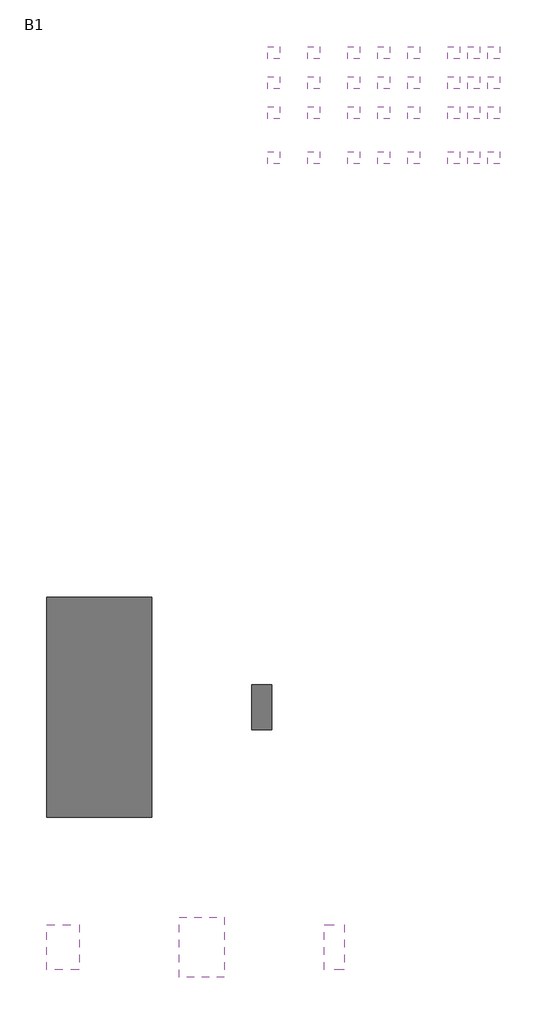
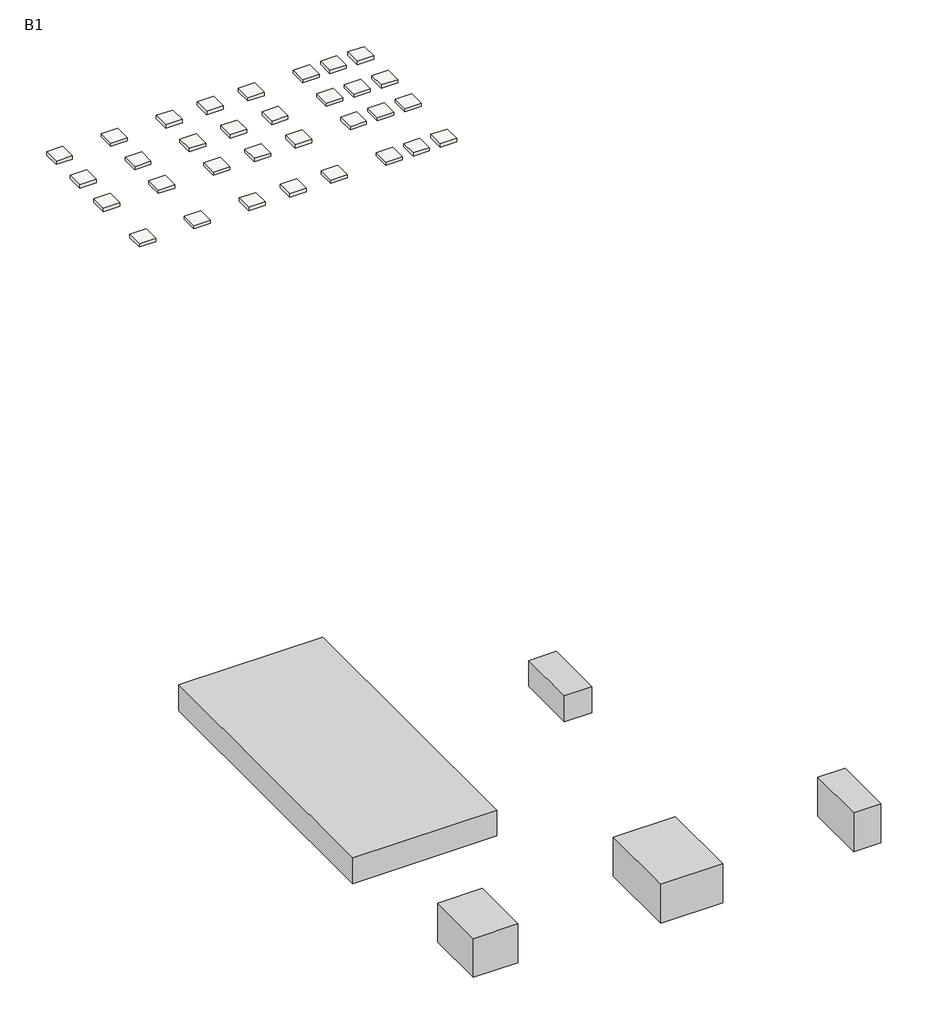
# One storey: 32 slabs, 5 proxies.
"""IFC4 building model written with IfcOpenShell, lengths in millimetres."""

import ifcopenshell
import ifcopenshell.guid

model = None  # the IFC model being written
_history = None  # IfcOwnerHistory: only IFC2X3 demands one
_inside = {}  # id of a spatial element -> (the spatial element, [elements in it])
_under = {}  # id of a project, library or spatial element -> (it, [spatial elements below it])
_declared = {}  # id of a project -> (the project, [libraries it declares])
_typed = {}  # id of a type object -> (the type object, [elements of that type])
_made_of = {}  # id of a material, layer set ... -> (it, [elements and type objects made of it])


def new_model(schema):
    """Start an empty IFC model of exactly this schema.

    Asked for "IFC4X3", IfcOpenShell would pick the latest addendum, in which some entities
    have other attributes; the version numbers below select the first issue.
    IFC2X3 requires an IfcOwnerHistory on every rooted entity: one is made here for all.
    """
    global model, _history
    if schema == "IFC4X3":
        model = ifcopenshell.file(schema_version=(4, 3, 0, 0))
    else:
        model = ifcopenshell.file(schema=schema)
    _inside.clear()
    _under.clear()
    _declared.clear()
    _typed.clear()
    _made_of.clear()
    _history = None
    if model.schema == "IFC2X3":
        org = make("IfcOrganization", Name="unknown")
        user = make(
            "IfcPersonAndOrganization",
            ThePerson=make("IfcPerson", FamilyName="unknown"),
            TheOrganization=org,
        )
        app = make(
            "IfcApplication",
            ApplicationDeveloper=org,
            Version="unknown",
            ApplicationFullName="unknown",
            ApplicationIdentifier="unknown",
        )
        _history = make(
            "IfcOwnerHistory",
            OwningUser=user,
            OwningApplication=app,
            ChangeAction="ADDED",
            CreationDate=0,
        )
    return model


def make(cls, **values):
    """One entity of the class cls with the attributes given. An attribute that is None is left unset."""
    return model.create_entity(
        cls, **{name: value for name, value in values.items() if value is not None}
    )


def rooted(cls, **values):
    """An entity with a GlobalId (a new one), such as an element, a storey or a relation."""
    return make(cls, GlobalId=ifcopenshell.guid.new(), OwnerHistory=_history, **values)


def si_unit(unit_type, name, prefix=None):
    """IfcSIUnit, for example si_unit("LENGTHUNIT", "METRE", prefix="MILLI")."""
    return make("IfcSIUnit", UnitType=unit_type, Prefix=prefix, Name=name)


def assignment(units):
    """IfcUnitAssignment: the units of a project."""
    return None if units is None else make("IfcUnitAssignment", Units=units)


def point(xyz):
    """IfcCartesianPoint."""
    return None if xyz is None else make("IfcCartesianPoint", Coordinates=xyz)


def direction(xyz):
    """IfcDirection."""
    return None if xyz is None else make("IfcDirection", DirectionRatios=xyz)


def frame(location, z_axis=None, x_axis=None):
    """IfcAxis2Placement3D, a coordinate frame: its origin and axes. An axis left out is left unset."""
    return make(
        "IfcAxis2Placement3D",
        Location=point(location),
        Axis=direction(z_axis),
        RefDirection=direction(x_axis),
    )


def origin():
    """The frame at (0, 0, 0) with its axes left unset."""
    return frame((0.0, 0.0, 0.0))


def origin_with_axes():
    """The frame at (0, 0, 0) with the z axis (0, 0, 1) and the x axis (1, 0, 0) written out."""
    return frame((0.0, 0.0, 0.0), z_axis=(0.0, 0.0, 1.0), x_axis=(1.0, 0.0, 0.0))


def place(relative_to, where):
    """IfcLocalPlacement: puts the frame where relative to a parent placement (None: the world)."""
    return make(
        "IfcLocalPlacement", PlacementRelTo=relative_to, RelativePlacement=where
    )


def context(
    kind, dimensions, precision=None, world=None, true_north=None, identifier=None
):
    """IfcGeometricRepresentationContext, for example the 3D "Model" context."""
    return make(
        "IfcGeometricRepresentationContext",
        ContextIdentifier=identifier,
        ContextType=kind,
        CoordinateSpaceDimension=dimensions,
        Precision=precision,
        WorldCoordinateSystem=world,
        TrueNorth=true_north,
    )


def project(units=None, contexts=None):
    """IfcProject with its units and contexts."""
    return rooted(
        "IfcProject",
        Name="project",
        RepresentationContexts=contexts,
        UnitsInContext=assignment(units),
    )


def spatial(cls, under=None, at=None, **own):
    """A site, building, storey or space (cls), placed at a placement, below another one or the project."""
    s = rooted(cls, ObjectPlacement=at, **own)
    if under is not None:
        _under.setdefault(under.id(), (under, []))[1].append(s)
    return s


def polyline(points):
    """IfcPolyline through the points."""
    return make("IfcPolyline", Points=[point(p) for p in points])


def outline(outer, holes=None, kind="AREA"):
    """IfcArbitraryClosedProfileDef: a profile drawn as a closed curve; with holes, ...WithVoids."""
    if holes is None:
        return make("IfcArbitraryClosedProfileDef", ProfileType=kind, OuterCurve=outer)
    return make(
        "IfcArbitraryProfileDefWithVoids",
        ProfileType=kind,
        OuterCurve=outer,
        InnerCurves=holes,
    )


def extrude(swept, where, along, depth):
    """IfcExtrudedAreaSolid: the profile swept, set in the frame where, extruded along a direction by depth."""
    return make(
        "IfcExtrudedAreaSolid",
        SweptArea=swept,
        Position=where,
        ExtrudedDirection=direction(along),
        Depth=depth,
    )


def shape(context_of_items, identifier, shape_type, items):
    """IfcShapeRepresentation: the items that make up one representation, for example the "Body"."""
    return make(
        "IfcShapeRepresentation",
        ContextOfItems=context_of_items,
        RepresentationIdentifier=identifier,
        RepresentationType=shape_type,
        Items=items,
    )


def source(mapping_origin, context_of_items, identifier, shape_type, items):
    """IfcRepresentationMap: a shape defined once, which mapped items show again and again."""
    return make(
        "IfcRepresentationMap",
        MappingOrigin=mapping_origin,
        MappedRepresentation=shape(context_of_items, identifier, shape_type, items),
    )


def transform(
    local_origin,
    x_axis=None,
    y_axis=None,
    z_axis=None,
    scale=None,
    scale2=None,
    scale3=None,
    uniform=True,
):
    """IfcCartesianTransformationOperator3D, or its non-uniform kind. x_axis, y_axis, z_axis: its Axis1, 2, 3."""
    if uniform:
        return make(
            "IfcCartesianTransformationOperator3D",
            Axis1=direction(x_axis),
            Axis2=direction(y_axis),
            LocalOrigin=point(local_origin),
            Scale=scale,
            Axis3=direction(z_axis),
        )
    return make(
        "IfcCartesianTransformationOperator3DnonUniform",
        Axis1=direction(x_axis),
        Axis2=direction(y_axis),
        LocalOrigin=point(local_origin),
        Scale=scale,
        Axis3=direction(z_axis),
        Scale2=scale2,
        Scale3=scale3,
    )


def mapped(mapping_source, mapping_target):
    """IfcMappedItem: shows the shape of a source again, moved by a transform."""
    return make(
        "IfcMappedItem", MappingSource=mapping_source, MappingTarget=mapping_target
    )


def made_of(thing, what):
    """Note that an element or type object is made of a material, layer set ...; save() writes the relation."""
    if what is not None:
        _made_of.setdefault(what.id(), (what, []))[1].append(thing)
    return thing


def element(
    cls,
    number,
    at=None,
    inside=None,
    cuts=None,
    type_object=None,
    material=None,
    context=None,
    identifier="Body",
    shape_type=None,
    held_by="IfcProductDefinitionShape",
    body=None,
    shapes=None,
    **own,
):
    """One element of the class cls, such as IfcWall. Its Tag is "e" and its number.

    at: its placement. inside: the storey or other place that contains it. cuts: it is an
    opening in that element (IfcRelVoidsElement). A single representation is given by context,
    identifier, shape_type and body (its items); several are given by shapes. held_by: the class
    of the entity that holds the representations. save() writes the other relations.
    """
    e = rooted(cls, Tag="e%d" % number, ObjectPlacement=at, **own)
    if body is not None:
        shapes = [shape(context, identifier, shape_type, body)]
    if shapes is not None:
        e.Representation = make(held_by, Representations=shapes)
    if inside is not None:
        _inside.setdefault(inside.id(), (inside, []))[1].append(e)
    if cuts is not None:
        rooted(
            "IfcRelVoidsElement", RelatingBuildingElement=cuts, RelatedOpeningElement=e
        )
    if type_object is not None:
        _typed.setdefault(type_object.id(), (type_object, []))[1].append(e)
    return made_of(e, material)


def aggregate(whole, parts):
    """IfcRelAggregates: a whole, such as a stair, and the parts it consists of."""
    return rooted("IfcRelAggregates", RelatingObject=whole, RelatedObjects=parts)


def save(model, path):
    """Write the relations noted so far, then the file.

    IfcRelAggregates (storeys below a building ...), IfcRelContainedInSpatialStructure (elements
    in a storey), IfcRelDefinesByType, IfcRelAssociatesMaterial and IfcRelDeclares: one each for
    every whole, place, type object, material and project.
    """
    for whole, parts in _under.values():
        aggregate(whole, parts)
    for where, things in _inside.values():
        rooted(
            "IfcRelContainedInSpatialStructure",
            RelatedElements=things,
            RelatingStructure=where,
        )
    for kind, things in _typed.values():
        rooted("IfcRelDefinesByType", RelatedObjects=things, RelatingType=kind)
    for what, things in _made_of.values():
        rooted("IfcRelAssociatesMaterial", RelatedObjects=things, RelatingMaterial=what)
    for by, libraries in _declared.values():
        rooted("IfcRelDeclares", RelatingContext=by, RelatedDefinitions=libraries)
    model.write(path)


def generic_models_1d705098(model_context):
    return source(origin(), model_context, "Body", "SweptSolid", [
        extrude(outline(polyline([(3250.0, 4500.0), (3250.0, -4500.0), (-3250.0, -4500.0), (-3250.0, 4500.0), (3250.0, 4500.0)])), origin_with_axes(), (0.0, 0.0, 1.0), 6000.0),
    ])


def generic_models_399a6151(model_context):
    return source(origin(), model_context, "Body", "SweptSolid", [
        extrude(outline(polyline([(4500.0, 6000.0), (4500.0, -6000.0), (-4500.0, -6000.0), (-4500.0, 6000.0), (4500.0, 6000.0)])), origin_with_axes(), (0.0, 0.0, 1.0), 6000.0),
    ])


def generic_models_29bcd6f9(model_context):
    return source(origin(), model_context, "Body", "SweptSolid", [
        extrude(outline(polyline([(2000.0, 4500.0), (2000.0, -4500.0), (-2000.0, -4500.0), (-2000.0, 4500.0), (2000.0, 4500.0)])), origin_with_axes(), (0.0, 0.0, 1.0), 6000.0),
    ])


def generic_models_a454a2aa(model_context):
    return source(origin(), model_context, "Body", "SweptSolid", [
        extrude(outline(polyline([(10500.0, 22000.0), (10500.0, -22000.0), (-10500.0, -22000.0), (-10500.0, 22000.0), (10500.0, 22000.0)])), origin_with_axes(), (0.0, 0.0, 1.0), 4000.0),
    ])


def generic_models_73802227(model_context):
    return source(origin(), model_context, "Body", "SweptSolid", [
        extrude(outline(polyline([(2000.0, 4500.0), (2000.0, -4500.0), (-2000.0, -4500.0), (-2000.0, 4500.0), (2000.0, 4500.0)])), origin_with_axes(), (0.0, 0.0, 1.0), 4000.0),
    ])


def ft112_footing_rectangular_ft112_2400x2400x500_5fe39465(model_context):
    return source(origin(), model_context, "Body", "SweptSolid", [
        extrude(outline(polyline([(1200.0, 1200.0), (1200.0, -1200.0), (-1200.0, -1200.0), (-1200.0, 1200.0), (1200.0, 1200.0)])), frame((0.0, 0.0, -500.0), z_axis=(0.0, 0.0, 1.0), x_axis=(1.0, 0.0, 0.0)), (0.0, 0.0, 1.0), 500.0),
    ])


model = new_model("IFC4")

# Units and contexts
model_context = context("Model", 3, world=origin())
ifc_project = project(units=[si_unit("LENGTHUNIT", "METRE", prefix="MILLI")], contexts=[model_context])

# Site, building, storey
site = spatial("IfcSite", under=ifc_project)
building = spatial("IfcBuilding", under=site)
storey = spatial("IfcBuildingStorey", under=building, Name="B1", Elevation=-4000.0)

# Proxies
placement = place(None, origin())
generic_models_shape = generic_models_1d705098(model_context)
element("IfcBuildingElementProxy", 1, Name="Space Planning Box_hec : Space Planning Box_hec", ObjectType="Space Planning Box_hec : Space Planning Box_hec", at=placement, inside=storey, context=model_context, shape_type="MappedRepresentation", body=[
    mapped(generic_models_shape, transform((3250.0, 6000.0, 0.0), x_axis=(1.0, 0.0, 0.0), y_axis=(0.0, 1.0, 0.0), z_axis=(0.0, 0.0, 1.0))),
])
generic_models_2_shape = generic_models_399a6151(model_context)
element("IfcBuildingElementProxy", 2, Name="Space Planning Box_hec : Space Planning Box_hec", ObjectType="Space Planning Box_hec : Space Planning Box_hec", at=placement, inside=storey, context=model_context, shape_type="MappedRepresentation", body=[
    mapped(generic_models_2_shape, transform((31000.0, 6000.0, 0.0), x_axis=(1.0, 0.0, 0.0), y_axis=(0.0, 1.0, 0.0), z_axis=(0.0, 0.0, 1.0))),
])
generic_models_3_shape = generic_models_29bcd6f9(model_context)
element("IfcBuildingElementProxy", 3, Name="Space Planning Box_hec : Space Planning Box_hec", ObjectType="Space Planning Box_hec : Space Planning Box_hec", at=placement, inside=storey, context=model_context, shape_type="MappedRepresentation", body=[
    mapped(generic_models_3_shape, transform((57500.0, 6000.0, 0.0), x_axis=(1.0, 0.0, 0.0), y_axis=(0.0, 1.0, 0.0), z_axis=(0.0, 0.0, 1.0))),
])
generic_models_4_shape = generic_models_a454a2aa(model_context)
element("IfcBuildingElementProxy", 4, Name="Space Planning Box_hec : Space Planning Box_hec", ObjectType="Space Planning Box_hec : Space Planning Box_hec", at=placement, inside=storey, context=model_context, shape_type="MappedRepresentation", body=[
    mapped(generic_models_4_shape, transform((10500.0, 54000.0, -4000.0), x_axis=(1.0, 0.0, 0.0), y_axis=(0.0, 1.0, 0.0), z_axis=(0.0, 0.0, 1.0))),
])
generic_models_5_shape = generic_models_73802227(model_context)
element("IfcBuildingElementProxy", 5, Name="Space Planning Box_hec : Space Planning Box_hec", ObjectType="Space Planning Box_hec : Space Planning Box_hec", at=placement, inside=storey, context=model_context, shape_type="MappedRepresentation", body=[
    mapped(generic_models_5_shape, transform((43000.0, 54000.0, -4000.0), x_axis=(1.0, 0.0, 0.0), y_axis=(0.0, 1.0, 0.0), z_axis=(0.0, 0.0, 1.0))),
])

# Slabs
ft112_footing_rectangular_ft112_2400x2400x500_shape = ft112_footing_rectangular_ft112_2400x2400x500_5fe39465(model_context)
element("IfcSlab", 6, ObjectType="FT112-Footing-Rectangular : FT112_2400x2400x500", at=placement, inside=storey, context=model_context, shape_type="MappedRepresentation", body=[
    mapped(ft112_footing_rectangular_ft112_2400x2400x500_shape, transform((45459.6521483, 184923.8614395, 0.0), x_axis=(1.0, 0.0, 0.0), y_axis=(0.0, 1.0, 0.0), z_axis=(0.0, 0.0, 1.0))),
])
element("IfcSlab", 7, ObjectType="FT112-Footing-Rectangular : FT112_2400x2400x500", at=placement, inside=storey, context=model_context, shape_type="MappedRepresentation", body=[
    mapped(ft112_footing_rectangular_ft112_2400x2400x500_shape, transform((45459.6521483, 178923.8614395, 0.0), x_axis=(1.0, 0.0, 0.0), y_axis=(0.0, 1.0, 0.0), z_axis=(0.0, 0.0, 1.0))),
])
element("IfcSlab", 8, ObjectType="FT112-Footing-Rectangular : FT112_2400x2400x500", at=placement, inside=storey, context=model_context, shape_type="MappedRepresentation", body=[
    mapped(ft112_footing_rectangular_ft112_2400x2400x500_shape, transform((45459.6521483, 172923.8614395, 0.0), x_axis=(1.0, 0.0, 0.0), y_axis=(0.0, 1.0, 0.0), z_axis=(0.0, 0.0, 1.0))),
])
element("IfcSlab", 9, ObjectType="FT112-Footing-Rectangular : FT112_2400x2400x500", at=placement, inside=storey, context=model_context, shape_type="MappedRepresentation", body=[
    mapped(ft112_footing_rectangular_ft112_2400x2400x500_shape, transform((45459.6521483, 163923.8614395, 0.0), x_axis=(1.0, 0.0, 0.0), y_axis=(0.0, 1.0, 0.0), z_axis=(0.0, 0.0, 1.0))),
])
element("IfcSlab", 10, ObjectType="FT112-Footing-Rectangular : FT112_2400x2400x500", at=placement, inside=storey, context=model_context, shape_type="MappedRepresentation", body=[
    mapped(ft112_footing_rectangular_ft112_2400x2400x500_shape, transform((53459.6521483, 184923.8614395, 0.0), x_axis=(1.0, 0.0, 0.0), y_axis=(0.0, 1.0, 0.0), z_axis=(0.0, 0.0, 1.0))),
])
element("IfcSlab", 11, ObjectType="FT112-Footing-Rectangular : FT112_2400x2400x500", at=placement, inside=storey, context=model_context, shape_type="MappedRepresentation", body=[
    mapped(ft112_footing_rectangular_ft112_2400x2400x500_shape, transform((53459.6521483, 178923.8614395, 0.0), x_axis=(1.0, 0.0, 0.0), y_axis=(0.0, 1.0, 0.0), z_axis=(0.0, 0.0, 1.0))),
])
element("IfcSlab", 12, ObjectType="FT112-Footing-Rectangular : FT112_2400x2400x500", at=placement, inside=storey, context=model_context, shape_type="MappedRepresentation", body=[
    mapped(ft112_footing_rectangular_ft112_2400x2400x500_shape, transform((53459.6521483, 172923.8614395, 0.0), x_axis=(1.0, 0.0, 0.0), y_axis=(0.0, 1.0, 0.0), z_axis=(0.0, 0.0, 1.0))),
])
element("IfcSlab", 13, ObjectType="FT112-Footing-Rectangular : FT112_2400x2400x500", at=placement, inside=storey, context=model_context, shape_type="MappedRepresentation", body=[
    mapped(ft112_footing_rectangular_ft112_2400x2400x500_shape, transform((53459.6521483, 163923.8614395, 0.0), x_axis=(1.0, 0.0, 0.0), y_axis=(0.0, 1.0, 0.0), z_axis=(0.0, 0.0, 1.0))),
])
element("IfcSlab", 14, ObjectType="FT112-Footing-Rectangular : FT112_2400x2400x500", at=placement, inside=storey, context=model_context, shape_type="MappedRepresentation", body=[
    mapped(ft112_footing_rectangular_ft112_2400x2400x500_shape, transform((61459.6521483, 184923.8614395, 0.0), x_axis=(1.0, 0.0, 0.0), y_axis=(0.0, 1.0, 0.0), z_axis=(0.0, 0.0, 1.0))),
])
element("IfcSlab", 15, ObjectType="FT112-Footing-Rectangular : FT112_2400x2400x500", at=placement, inside=storey, context=model_context, shape_type="MappedRepresentation", body=[
    mapped(ft112_footing_rectangular_ft112_2400x2400x500_shape, transform((61459.6521483, 178923.8614395, 0.0), x_axis=(1.0, 0.0, 0.0), y_axis=(0.0, 1.0, 0.0), z_axis=(0.0, 0.0, 1.0))),
])
element("IfcSlab", 16, ObjectType="FT112-Footing-Rectangular : FT112_2400x2400x500", at=placement, inside=storey, context=model_context, shape_type="MappedRepresentation", body=[
    mapped(ft112_footing_rectangular_ft112_2400x2400x500_shape, transform((61459.6521483, 172923.8614395, 0.0), x_axis=(1.0, 0.0, 0.0), y_axis=(0.0, 1.0, 0.0), z_axis=(0.0, 0.0, 1.0))),
])
element("IfcSlab", 17, ObjectType="FT112-Footing-Rectangular : FT112_2400x2400x500", at=placement, inside=storey, context=model_context, shape_type="MappedRepresentation", body=[
    mapped(ft112_footing_rectangular_ft112_2400x2400x500_shape, transform((61459.6521483, 163923.8614395, 0.0), x_axis=(1.0, 0.0, 0.0), y_axis=(0.0, 1.0, 0.0), z_axis=(0.0, 0.0, 1.0))),
])
element("IfcSlab", 18, ObjectType="FT112-Footing-Rectangular : FT112_2400x2400x500", at=placement, inside=storey, context=model_context, shape_type="MappedRepresentation", body=[
    mapped(ft112_footing_rectangular_ft112_2400x2400x500_shape, transform((67459.6521483, 184923.8614395, 0.0), x_axis=(1.0, 0.0, 0.0), y_axis=(0.0, 1.0, 0.0), z_axis=(0.0, 0.0, 1.0))),
])
element("IfcSlab", 19, ObjectType="FT112-Footing-Rectangular : FT112_2400x2400x500", at=placement, inside=storey, context=model_context, shape_type="MappedRepresentation", body=[
    mapped(ft112_footing_rectangular_ft112_2400x2400x500_shape, transform((67459.6521483, 178923.8614395, 0.0), x_axis=(1.0, 0.0, 0.0), y_axis=(0.0, 1.0, 0.0), z_axis=(0.0, 0.0, 1.0))),
])
element("IfcSlab", 20, ObjectType="FT112-Footing-Rectangular : FT112_2400x2400x500", at=placement, inside=storey, context=model_context, shape_type="MappedRepresentation", body=[
    mapped(ft112_footing_rectangular_ft112_2400x2400x500_shape, transform((67459.6521483, 172923.8614395, 0.0), x_axis=(1.0, 0.0, 0.0), y_axis=(0.0, 1.0, 0.0), z_axis=(0.0, 0.0, 1.0))),
])
element("IfcSlab", 21, ObjectType="FT112-Footing-Rectangular : FT112_2400x2400x500", at=placement, inside=storey, context=model_context, shape_type="MappedRepresentation", body=[
    mapped(ft112_footing_rectangular_ft112_2400x2400x500_shape, transform((67459.6521483, 163923.8614395, 0.0), x_axis=(1.0, 0.0, 0.0), y_axis=(0.0, 1.0, 0.0), z_axis=(0.0, 0.0, 1.0))),
])
element("IfcSlab", 22, ObjectType="FT112-Footing-Rectangular : FT112_2400x2400x500", at=placement, inside=storey, context=model_context, shape_type="MappedRepresentation", body=[
    mapped(ft112_footing_rectangular_ft112_2400x2400x500_shape, transform((73459.6521483, 184923.8614395, 0.0), x_axis=(1.0, 0.0, 0.0), y_axis=(0.0, 1.0, 0.0), z_axis=(0.0, 0.0, 1.0))),
])
element("IfcSlab", 23, ObjectType="FT112-Footing-Rectangular : FT112_2400x2400x500", at=placement, inside=storey, context=model_context, shape_type="MappedRepresentation", body=[
    mapped(ft112_footing_rectangular_ft112_2400x2400x500_shape, transform((73459.6521483, 178923.8614395, 0.0), x_axis=(1.0, 0.0, 0.0), y_axis=(0.0, 1.0, 0.0), z_axis=(0.0, 0.0, 1.0))),
])
element("IfcSlab", 24, ObjectType="FT112-Footing-Rectangular : FT112_2400x2400x500", at=placement, inside=storey, context=model_context, shape_type="MappedRepresentation", body=[
    mapped(ft112_footing_rectangular_ft112_2400x2400x500_shape, transform((73459.6521483, 172923.8614395, 0.0), x_axis=(1.0, 0.0, 0.0), y_axis=(0.0, 1.0, 0.0), z_axis=(0.0, 0.0, 1.0))),
])
element("IfcSlab", 25, ObjectType="FT112-Footing-Rectangular : FT112_2400x2400x500", at=placement, inside=storey, context=model_context, shape_type="MappedRepresentation", body=[
    mapped(ft112_footing_rectangular_ft112_2400x2400x500_shape, transform((73459.6521483, 163923.8614395, 0.0), x_axis=(1.0, 0.0, 0.0), y_axis=(0.0, 1.0, 0.0), z_axis=(0.0, 0.0, 1.0))),
])
element("IfcSlab", 26, ObjectType="FT112-Footing-Rectangular : FT112_2400x2400x500", at=placement, inside=storey, context=model_context, shape_type="MappedRepresentation", body=[
    mapped(ft112_footing_rectangular_ft112_2400x2400x500_shape, transform((81459.6521483, 184923.8614395, 0.0), x_axis=(1.0, 0.0, 0.0), y_axis=(0.0, 1.0, 0.0), z_axis=(0.0, 0.0, 1.0))),
])
element("IfcSlab", 27, ObjectType="FT112-Footing-Rectangular : FT112_2400x2400x500", at=placement, inside=storey, context=model_context, shape_type="MappedRepresentation", body=[
    mapped(ft112_footing_rectangular_ft112_2400x2400x500_shape, transform((81459.6521483, 178923.8614395, 0.0), x_axis=(1.0, 0.0, 0.0), y_axis=(0.0, 1.0, 0.0), z_axis=(0.0, 0.0, 1.0))),
])
element("IfcSlab", 28, ObjectType="FT112-Footing-Rectangular : FT112_2400x2400x500", at=placement, inside=storey, context=model_context, shape_type="MappedRepresentation", body=[
    mapped(ft112_footing_rectangular_ft112_2400x2400x500_shape, transform((81459.6521483, 172923.8614395, 0.0), x_axis=(1.0, 0.0, 0.0), y_axis=(0.0, 1.0, 0.0), z_axis=(0.0, 0.0, 1.0))),
])
element("IfcSlab", 29, ObjectType="FT112-Footing-Rectangular : FT112_2400x2400x500", at=placement, inside=storey, context=model_context, shape_type="MappedRepresentation", body=[
    mapped(ft112_footing_rectangular_ft112_2400x2400x500_shape, transform((81459.6521483, 163923.8614395, 0.0), x_axis=(1.0, 0.0, 0.0), y_axis=(0.0, 1.0, 0.0), z_axis=(0.0, 0.0, 1.0))),
])
element("IfcSlab", 30, ObjectType="FT112-Footing-Rectangular : FT112_2400x2400x500", at=placement, inside=storey, context=model_context, shape_type="MappedRepresentation", body=[
    mapped(ft112_footing_rectangular_ft112_2400x2400x500_shape, transform((85459.6521483, 184923.8614395, 0.0), x_axis=(1.0, 0.0, 0.0), y_axis=(0.0, 1.0, 0.0), z_axis=(0.0, 0.0, 1.0))),
])
element("IfcSlab", 31, ObjectType="FT112-Footing-Rectangular : FT112_2400x2400x500", at=placement, inside=storey, context=model_context, shape_type="MappedRepresentation", body=[
    mapped(ft112_footing_rectangular_ft112_2400x2400x500_shape, transform((85459.6521483, 178923.8614395, 0.0), x_axis=(1.0, 0.0, 0.0), y_axis=(0.0, 1.0, 0.0), z_axis=(0.0, 0.0, 1.0))),
])
element("IfcSlab", 32, ObjectType="FT112-Footing-Rectangular : FT112_2400x2400x500", at=placement, inside=storey, context=model_context, shape_type="MappedRepresentation", body=[
    mapped(ft112_footing_rectangular_ft112_2400x2400x500_shape, transform((85459.6521483, 172923.8614395, 0.0), x_axis=(1.0, 0.0, 0.0), y_axis=(0.0, 1.0, 0.0), z_axis=(0.0, 0.0, 1.0))),
])
element("IfcSlab", 33, ObjectType="FT112-Footing-Rectangular : FT112_2400x2400x500", at=placement, inside=storey, context=model_context, shape_type="MappedRepresentation", body=[
    mapped(ft112_footing_rectangular_ft112_2400x2400x500_shape, transform((85459.6521483, 163923.8614395, 0.0), x_axis=(1.0, 0.0, 0.0), y_axis=(0.0, 1.0, 0.0), z_axis=(0.0, 0.0, 1.0))),
])
element("IfcSlab", 34, ObjectType="FT112-Footing-Rectangular : FT112_2400x2400x500", at=placement, inside=storey, context=model_context, shape_type="MappedRepresentation", body=[
    mapped(ft112_footing_rectangular_ft112_2400x2400x500_shape, transform((89459.6521483, 184923.8614395, 0.0), x_axis=(1.0, 0.0, 0.0), y_axis=(0.0, 1.0, 0.0), z_axis=(0.0, 0.0, 1.0))),
])
element("IfcSlab", 35, ObjectType="FT112-Footing-Rectangular : FT112_2400x2400x500", at=placement, inside=storey, context=model_context, shape_type="MappedRepresentation", body=[
    mapped(ft112_footing_rectangular_ft112_2400x2400x500_shape, transform((89459.6521483, 178923.8614395, 0.0), x_axis=(1.0, 0.0, 0.0), y_axis=(0.0, 1.0, 0.0), z_axis=(0.0, 0.0, 1.0))),
])
element("IfcSlab", 36, ObjectType="FT112-Footing-Rectangular : FT112_2400x2400x500", at=placement, inside=storey, context=model_context, shape_type="MappedRepresentation", body=[
    mapped(ft112_footing_rectangular_ft112_2400x2400x500_shape, transform((89459.6521483, 172923.8614395, 0.0), x_axis=(1.0, 0.0, 0.0), y_axis=(0.0, 1.0, 0.0), z_axis=(0.0, 0.0, 1.0))),
])
element("IfcSlab", 37, ObjectType="FT112-Footing-Rectangular : FT112_2400x2400x500", at=placement, inside=storey, context=model_context, shape_type="MappedRepresentation", body=[
    mapped(ft112_footing_rectangular_ft112_2400x2400x500_shape, transform((89459.6521483, 163923.8614395, 0.0), x_axis=(1.0, 0.0, 0.0), y_axis=(0.0, 1.0, 0.0), z_axis=(0.0, 0.0, 1.0))),
])

save(model, "model.ifc")

# Revit data of these elements
# Project information
#   Building Name = "MAIN GATE SECURITY BUILDING"
#   Project Status = "Project Status"
#   Client Name = "현대엔지니어링"
#   Project Address = "서울시 종로구 율곡로 75(계동)"
#   Project Name = "Therma Visayas Energy Project"
#   Project Number = "-"
# Grids (mm)
#   "A": line (45459.652, 190234.526) -> (45459.652, 152139.384)
#   "B": line (53459.652, 190234.526) -> (53459.652, 152139.384)
#   "C": line (61459.652, 190234.526) -> (61459.652, 152139.384)
#   "D": line (67459.652, 190234.526) -> (67459.652, 152139.384)
#   "E": line (73459.652, 190234.526) -> (73459.652, 152139.384)
#   "F": line (81459.652, 190234.526) -> (81459.652, 152139.384)
#   "G": line (85459.652, 190234.526) -> (85459.652, 152139.384)
#   "H": line (89459.652, 190234.526) -> (89459.652, 152139.384)
#   "4": line (39389.066, 184923.861) -> (95952.222, 184923.861)
#   "3": line (39389.066, 178923.861) -> (95952.222, 178923.861)
#   "2": line (39389.066, 172923.861) -> (95952.222, 172923.861)
#   "1": line (39389.066, 163923.861) -> (95952.222, 163923.861)
# Type "Space Planning Box_hec : Space Planning Box_hec"
#   Type Comments = "..."
#   Room Name [instance default] = "?"
#   Interior Finish [instance default] = ""
#   Exterior Finish [instance default] = ""
#   Department [instance default] = ""
#   Assembly Code = "..."
#   Width [instance default] = 1524 mm
#   Program Area [instance default] = 0.00 m²
#   Length [instance default] = 1524 mm
#   Height [instance default] = 1524 mm
#   Area [instance default] = 2.32258 m²
#   Fill Color [instance default] = Cyan
#   Default Elevation = 0
# Type "FT112-Footing-Rectangular : FT112_2400x2400x500"
#   Description = "UG Shallow Foundation"
#   Width = 2400 mm
#   Length = 2400 mm
#   Foundation Thickness = 500 mm
#   hec_material3 [instance default] = none
#   hec_material2 [instance default] = A03AE056-00001_Bitumen/Bituminous/Asphalt Coating
#   hec_material1 [instance default] = A03AC035-00001_Form Work (3 times in use)_Flat
#   Structural Material [instance default] = A03AC032-00007_Structural Concrete_Type1_25MPa-30Mpa
#   Assembly Code = ""
# Element 1 (IfcBuildingElementProxy, "Space Planning Box_hec : Space Planning Box_hec")
#   Room Name = "Switchgear Room"
#   Interior Finish = "IF1"
#   Exterior Finish = "EF1"
#   Department = "EL"
#   Width = 6500 mm
#   Program Area = 58.50 m²
#   Length = 9000 mm
#   Height = 6000 mm
#   Area = 58.50 m²
#   Fill Color = Blue
#   Phase Created = New Construction
#   Materials on its faces: "Blue"
# Element 2 (IfcBuildingElementProxy, "Space Planning Box_hec : Space Planning Box_hec")
#   Room Name = "Battery Room"
#   Interior Finish = "IF4"
#   Exterior Finish = "EF1"
#   Department = "EL"
#   Width = 9000 mm
#   Program Area = 108.00 m²
#   Length = 12000 mm
#   Height = 6000 mm
#   Area = 108.00 m²
#   Fill Color = Blue
#   Phase Created = New Construction
#   Materials on its faces: "Blue"
# Element 3 (IfcBuildingElementProxy, "Space Planning Box_hec : Space Planning Box_hec")
#   Room Name = "Stairway"
#   Interior Finish = "IF2"
#   Exterior Finish = "EF1"
#   Department = "AR"
#   Width = 4000 mm
#   Program Area = 36.00 m²
#   Length = 9000 mm
#   Height = 6000 mm
#   Area = 36.00 m²
#   Fill Color = Lavender
#   Phase Created = New Construction
#   Materials on its faces: "Lavender"
# Element 4 (IfcBuildingElementProxy, "Space Planning Box_hec : Space Planning Box_hec")
#   Room Name = "Cable Room"
#   Interior Finish = "IF1"
#   Exterior Finish = "EF1"
#   Department = "EL"
#   Width = 21000 mm
#   Program Area = 924.00 m²
#   Length = 44000 mm
#   Height = 4000 mm
#   Area = 924.00 m²
#   Fill Color = Blue
#   Phase Created = New Construction
#   Materials on its faces: "Blue"
# Element 5 (IfcBuildingElementProxy, "Space Planning Box_hec : Space Planning Box_hec")
#   Room Name = "Stairway"
#   Interior Finish = "IF2"
#   Exterior Finish = "EF1"
#   Department = "EL"
#   Width = 4000 mm
#   Program Area = 36.00 m²
#   Length = 9000 mm
#   Height = 4000 mm
#   Area = 36.00 m²
#   Fill Color = Blue
#   Phase Created = New Construction
#   Materials on its faces: "Blue"
# Elements 6, 7, 8, 9, 10, 11, 12, 13, 14, 15, 16, 17, 18, 19, 20, 21, 22, 23, 24, 25, 26, 27, 28, 29, 30, 31, 32, 33, 34, 35, 36, 37 (IfcSlab, "FT112-Footing-Rectangular : FT112_2400x2400x500")
#   Comments = ""
#   hec_material3 = none
#   hec_material2 = none
#   hec_material1 = none
#   Structural Material = 콘크리트 - 현장타설 콘크리트
#   Phase Created = New Construction
#   Materials on its faces: "콘크리트 - 현장타설 콘크리트"
# Materials
#   "Cyan": class "Generic", colour RGB 0 255 255, transparency 0.2, Cost = 0
#   "A03AE056-00001_Bitumen/Bituminous/Asphalt Coating": class "Generic", colour RGB 17 17 17, transparency 0, Description = "Damp-proofing", W00) Work Master Code = "A03AE056-00001", W01) Work Master_Lv1 = "Concrete Work", W02) Work Master_Lv2 = "Concrete Protective Coating (U/G)", W03) Work Master_Spec.1 = "Bitumen/Bituminous/Asphalt Coating", Cost = 0
#   "A03AC035-00001_Form Work (3 times in use)_Flat": class "Wood", colour RGB 149 120 74, transparency 0, Description = "Plywood", W00) Work Master Code = "A03AC035-00001", W01) Work Master_Lv1 = "Concrete Work", W02) Work Master_Lv2 = "Substructure Work", W03) Work Master_Spec.1 = "Form Work (3 times in use)", W04) Work Master_Spec.2 = "Flat Form", W05) Work Master_Spec.3 = "Dressed Lumber, Plywood or Steel Form(Wood Planks are not Allowed) incl. Chamfer", Cost = 0
#   "A03AC032-00007_Structural Concrete_Type1_25MPa-30Mpa": class "Concrete", colour RGB 176 176 176, transparency 0, Keynote = "09910.A1", Description = "Reinf. Conc.", W00) Work Master Code = "A03AC032-00007", W01) Work Master_Lv1 = "Concrete Work", W02) Work Master_Lv2 = "Substructure Work", W03) Work Master_Spec.1 = "Structural Concrete", W04) Work Master_Spec.2 = "Cement Type-1", W05) Work Master_Spec.3 = "25MPa < F'c (Cylinder Strength) ≤ 30MPa", Cost = 0
#   "Blue": class "Generic", colour RGB 0 0 255, transparency 0.2, Cost = 0
#   "Lavender": class "Generic", colour RGB 186 85 211, transparency 0.2, Cost = 0
#   "콘크리트 - 현장타설 콘크리트": class "콘크리트", colour RGB 192 192 192, transparency 0
